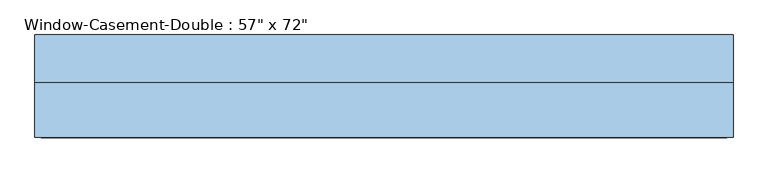
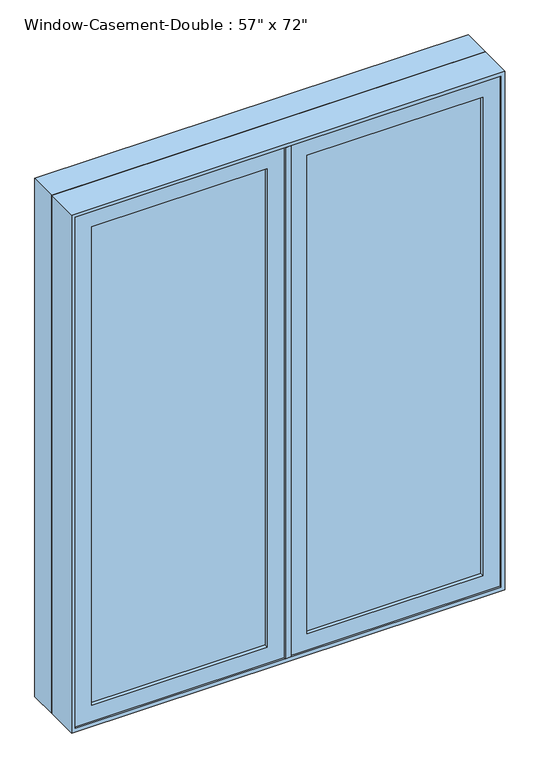
"""IFC4 building model written with IfcOpenShell, lengths in millimetres: window geometry."""

from ifc_helpers import new_model, si_unit, frame, origin, place, context, project, spatial, polyline, outline, extrude, faceted_brep, source, transform, mapped, element, save


def window_a1a4ced6(model_context):
    return source(origin(), model_context, "Body", "SolidModel", [
        faceted_brep([(9.525, -115.8875, 2730.5), (9.525, -65.0875, 2730.5), (-9.525, -65.0875, 2730.5), (-9.525, -115.8875, 2730.5), (9.525, -115.8875, 927.1), (-9.525, -115.8875, 927.1), (-9.525, -65.0875, 927.1), (9.525, -65.0875, 927.1), (-9.525, -65.0875, 2711.45), (-9.525, -65.0875, 946.15), (-30.1625, -65.0875, 2711.45), (-30.1625, -65.0875, 946.15), (-30.1625, -1.5875, 2711.45), (-30.1625, -1.5875, 946.15), (30.1625, -1.5875, 2711.45), (30.1625, -1.5875, 946.15), (30.1625, -65.0875, 2711.45), (30.1625, -65.0875, 946.15), (9.525, -65.0875, 2711.45), (9.525, -65.0875, 946.15)], [[[0, 1, 2, 3]], [[4, 5, 6, 7]], [[3, 5, 4, 0]], [[2, 8, 9, 6, 5, 3]], [[8, 10, 11, 9]], [[10, 12, 13, 11]], [[12, 14, 15, 13]], [[14, 16, 17, 15]], [[16, 18, 19, 17]], [[0, 4, 7, 19, 18, 1]], [[8, 2, 1, 18]], [[19, 7, 6, 9]], [[9, 11, 13, 15, 17, 19]], [[18, 16, 14, 12, 10, 8]]]),
        extrude(outline(polyline([(-66.675, -96.8375), (-654.05, -96.8375), (-654.05, -90.4875), (-66.675, -90.4875), (-66.675, -96.8375)])), frame((0.0, 0.0, 984.25), z_axis=(0.0, 0.0, 1.0), x_axis=(1.0, 0.0, 0.0)), (0.0, 0.0, 1.0), 1689.1),
        extrude(outline(polyline([(-654.05, -77.7875), (-66.675, -77.7875), (-66.675, -84.1375), (-654.05, -84.1375), (-654.05, -77.7875)])), frame((0.0, 0.0, 984.25), z_axis=(0.0, 0.0, 1.0), x_axis=(1.0, 0.0, 0.0)), (0.0, 0.0, 1.0), 1689.1),
        extrude(outline(polyline([(654.05, -96.8375), (66.675, -96.8375), (66.675, -90.4875), (654.05, -90.4875), (654.05, -96.8375)])), frame((0.0, 0.0, 984.25), z_axis=(0.0, 0.0, 1.0), x_axis=(1.0, 0.0, 0.0)), (0.0, 0.0, 1.0), 1689.1),
        extrude(outline(polyline([(66.675, -77.7875), (654.05, -77.7875), (654.05, -84.1375), (66.675, -84.1375), (66.675, -77.7875)])), frame((0.0, 0.0, 984.25), z_axis=(0.0, 0.0, 1.0), x_axis=(1.0, 0.0, 0.0)), (0.0, 0.0, 1.0), 1689.1),
        extrude(outline(polyline([(2730.5, -9.525), (2730.5, -711.2), (927.1, -711.2), (927.1, -9.525), (2730.5, -9.525)]), holes=[polyline([(2673.35, -654.05), (2673.35, -66.675), (984.25, -66.675), (984.25, -654.05), (2673.35, -654.05)])]), frame((0.0, -109.5375, 0.0), z_axis=(0.0, 1.0, 0.0), x_axis=(0.0, 0.0, 1.0)), (0.0, 0.0, 1.0), 44.45),
        extrude(outline(polyline([(927.1, 9.525), (927.1, 711.2), (2730.5, 711.2), (2730.5, 9.525), (927.1, 9.525)]), holes=[polyline([(984.25, 654.05), (984.25, 66.675), (2673.35, 66.675), (2673.35, 654.05), (984.25, 654.05)])]), frame((0.0, -109.5375, 0.0), z_axis=(0.0, 1.0, 0.0), x_axis=(0.0, 0.0, 1.0)), (0.0, 0.0, 1.0), 44.45),
        extrude(outline(polyline([(2743.2, -723.9), (914.4, -723.9), (914.4, 723.9), (2743.2, 723.9), (2743.2, -723.9)]), holes=[polyline([(2724.15, 704.85), (933.45, 704.85), (933.45, -704.85), (2724.15, -704.85), (2724.15, 704.85)])]), frame((0.0, -1.5875, 0.0), z_axis=(0.0, 1.0, 0.0), x_axis=(0.0, 0.0, 1.0)), (0.0, 0.0, 1.0), 98.425),
        faceted_brep([(692.15, -65.0875, 2711.45), (-692.15, -65.0875, 2711.45), (-692.15, -1.5875, 2711.45), (692.15, -1.5875, 2711.45), (711.2, -115.8875, 2730.5), (-711.2, -115.8875, 2730.5), (-711.2, -65.0875, 2730.5), (711.2, -65.0875, 2730.5), (723.9, -1.5875, 2743.2), (-723.9, -1.5875, 2743.2), (-723.9, -115.8875, 2743.2), (723.9, -115.8875, 2743.2), (-692.15, -65.0875, 946.15), (-692.15, -1.5875, 946.15), (-711.2, -115.8875, 927.1), (-711.2, -65.0875, 927.1), (-723.9, -1.5875, 914.4), (-723.9, -115.8875, 914.4), (692.15, -65.0875, 946.15), (692.15, -1.5875, 946.15), (711.2, -115.8875, 927.1), (711.2, -65.0875, 927.1), (723.9, -1.5875, 914.4), (723.9, -115.8875, 914.4)], [[[0, 1, 2, 3]], [[4, 5, 6, 7]], [[8, 9, 10, 11]], [[1, 12, 13, 2]], [[5, 14, 15, 6]], [[9, 16, 17, 10]], [[12, 18, 19, 13]], [[14, 20, 21, 15]], [[16, 22, 23, 17]], [[9, 8, 22, 16], [3, 2, 13, 19]], [[18, 0, 3, 19]], [[7, 6, 15, 21], [1, 0, 18, 12]], [[20, 4, 7, 21]], [[22, 8, 11, 23]], [[11, 10, 17, 23], [5, 4, 20, 14]]]),
    ])


if __name__ == "__main__":
    model = new_model("IFC4")
    model_context = context("Model", 3, world=origin())
    ifc_project = project(units=[si_unit("LENGTHUNIT", "METRE", prefix="MILLI")], contexts=[model_context])
    site = spatial("IfcSite", under=ifc_project)
    building = spatial("IfcBuilding", under=site)
    placement = place(None, origin())
    window_shape = window_a1a4ced6(model_context)
    element("IfcWindow", 1, ObjectType="Window-Casement-Double : 57\" x 72\"", at=placement, inside=building, context=model_context, shape_type="MappedRepresentation", body=[
        mapped(window_shape, transform((0.0, 0.0, 0.0), x_axis=(1.0, 0.0, 0.0), y_axis=(0.0, 1.0, 0.0), z_axis=(0.0, 0.0, 1.0))),
    ])
    save(model, "model.ifc")

# Revit data of these elements
# Type "Window-Casement-Double : 57\" x 72\""
#   Type Mark = "62"
#   Fire Rating = "0.5h"
#   Assembly Code = "B2020100"
#   Analytic Construction = "Double glazing - domestic"
#   Frame Extension [instance default] = 0' - 0 1/4"
#   Window Inset [instance default] = 0' - 0"
#   Wall Thickness [instance default] = 0' - 6"
#   Interior Wall Closure [instance default] = 0' - 2 1/4"
#   Half Width = 2' - 4 1/2"
#   Visual Light Transmittance = 0.81
#   Thermal Resistance (R) = 1.8146 (h·ft²·°F)/BTU
#   Solar Heat Gain Coefficient = 0.76
#   Rough Width = 4' - 9 1/2"
#   Rough Height = 6' - 0 1/2"
#   Height = 6' - 0"
#   Heat Transfer Coefficient (U) = 0.5511 BTU/(h·ft²·°F)
#   Exterior Wall Closure [instance default] = 0' - 1 1/4"
#   Extension Jamb [instance default] = 0' - 2 1/4"
#   Default Sill Height = 3' - 0"
#   Width = 4' - 9"
#   Define Thermal Properties by = 0
#   Muntin Visibility = yes
#   Interior Trim Visibility [instance default] = yes
#   Exterior Trim Visibility [instance default] = yes
#   Extension Jamb Visibility [instance default] = yes
#   Interior Trim Material = Wood - Stained
#   Muntin Pattern = Muntin Pattern_2x2 : Muntin Pattern_2x2
#   Interior Trim = Trim-Window-Interior-Flat : Picture Frame
#   Interior Frame Material = Wood - Stained
#   Glass Panel Material = Glass
#   Exterior Trim Material = Clad - White
#   Exterior Trim = Trim-Window-Exterior-Flat : with Sill
#   Exterior Frame Material = Clad - White
#   Wall Closure = (empty or 0)
# Element 1 (IfcWindow, "Window-Casement-Double : 57\" x 72\"")
#   Wall Thickness = 0' - 7 5/8"
#   Extension Jamb = 0' - 3 7/8"
#   Materials on its faces: "Wood - Stained", "Glass", "Clad - White"
# Materials
#   "Wood - Stained": class "Wood", colour RGB 224 178 126, transparency 0, Cost = 0
#   "Glass": class "Glass", colour RGB 236 240 239, transparency 0.5, Description = "Soda Lime Glass", Cost = 0
#   "Clad - White": class "Wood", colour RGB 216 216 204, transparency 0, Cost = 0
